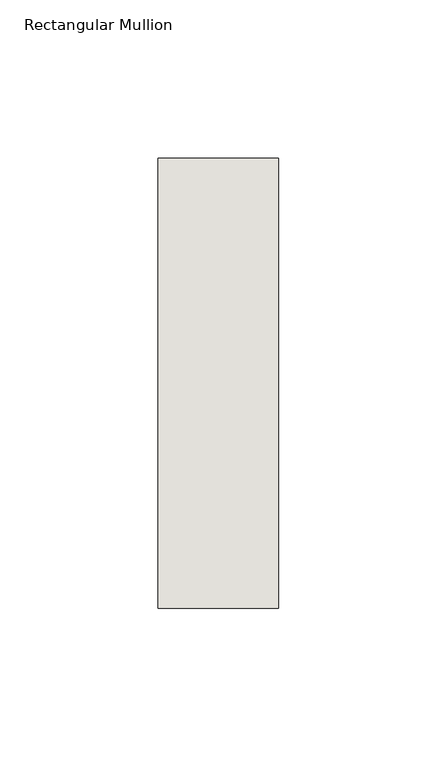
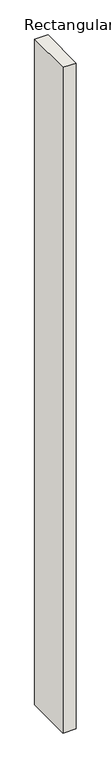
"""IFC4 building model written with IfcOpenShell, lengths in millimetres: wall geometry, Rectangular Mullion : NLRS_21_CWM_hsb-regel 38x142_gen_rsf."""

from ifc_helpers import new_model, si_unit, frame, origin, place, context, project, spatial, polyline, outline, extrude, source, transform, mapped, element, save


def rectangular_mullion_39366410(model_context):
    return source(origin(), model_context, "Body", "SweptSolid", [
        extrude(outline(polyline([(19.0, -71.0), (-19.0, -71.0), (-19.0, 71.0), (19.0, 71.0), (19.0, -71.0)])), frame((0.0, 0.0, -2038.0), z_axis=(0.0, 0.0, 1.0), x_axis=(1.0, 0.0, 0.0)), (0.0, 0.0, 1.0), 2038.0),
    ])


if __name__ == "__main__":
    model = new_model("IFC4")
    model_context = context("Model", 3, world=origin())
    ifc_project = project(units=[si_unit("LENGTHUNIT", "METRE", prefix="MILLI")], contexts=[model_context])
    site = spatial("IfcSite", under=ifc_project)
    building = spatial("IfcBuilding", under=site)
    placement = place(None, origin())
    rectangular_mullion_shape = rectangular_mullion_39366410(model_context)
    element("IfcWall", 1, ObjectType="Rectangular Mullion : NLRS_21_CWM_hsb-regel 38x142_gen_rsf", at=placement, inside=building, context=model_context, shape_type="MappedRepresentation", body=[
        mapped(rectangular_mullion_shape, transform((0.0, 0.0, 0.0), x_axis=(1.0, 0.0, 0.0), y_axis=(0.0, 1.0, 0.0), z_axis=(0.0, 0.0, 1.0))),
    ])
    save(model, "model.ifc")

# Revit data of these elements
# Type "Rectangular Mullion : NLRS_21_CWM_hsb-regel 38x142_gen_rsf"
#   Type IfcGUID = "07M7mRoiH1CR8m_RSKIwpF"
#   Assembly Code = "21.10"
#   IfcExportAs = "IfcWall"
#   built-in parameter 1007322 = 0.465879 (stored number, unit not read)
#   built-in parameter 1007321 = 0.062336 (stored number, unit not read)
#   built-in parameter 1007320 = 0.062336 (stored number, unit not read)
# Element 1 (IfcWall, "Rectangular Mullion : NLRS_21_CWM_hsb-regel 38x142_gen_rsf")
#   Materials on its faces: "NLRS_i2_hout naaldhout vuren_gen_rsf"
# Materials
#   "NLRS_i2_hout naaldhout vuren_gen_rsf": class "I - Hout", colour RGB 234 199 147, transparency 0, Keynote = "i2", Manufacturer = "Revit Standards Foundation", URL = "www.revitstandards.org", Description = "hout vuren", Cost = 0
